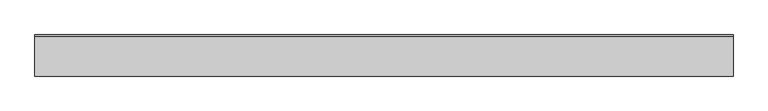
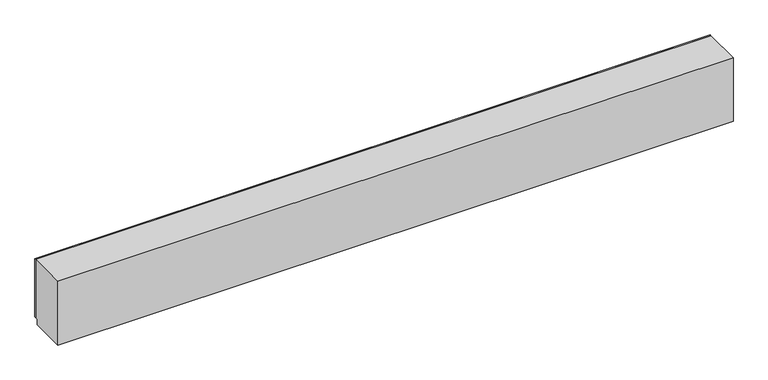
"""IFC4 building model written with IfcOpenShell, lengths in millimetres: furniture geometry, OD_CW_Base Cabinet : OD_CW_Base Cabinet."""

from ifc_helpers import new_model, si_unit, frame, origin, place, context, project, spatial, polyline, outline, extrude, source, transform, mapped, element, save


def furniture_ba198ac1(model_context):
    return source(origin(), model_context, "Body", "SweptSolid", [
        extrude(outline(polyline([(18.7377049, 82.55), (18.7377049, 107.95), (12195.519328, 107.95), (12195.519328, 82.55), (18.7377049, 82.55)])), frame((0.0, 0.0, 101.6), z_axis=(0.0, 0.0, 1.0), x_axis=(1.0, 0.0, 0.0)), (0.0, 0.0, 1.0), 1112.7587451),
        extrude(outline(polyline([(82.55, 1214.3587451), (82.55, 101.6), (31.75, 101.6), (31.75, 0.0), (-609.6, 0.0), (-609.6, 1214.3587451), (82.55, 1214.3587451)])), frame((18.7377049, 0.0, 0.0), z_axis=(1.0, 0.0, 0.0), x_axis=(0.0, 1.0, 0.0)), (0.0, 0.0, 1.0), 12176.7816231),
    ])


if __name__ == "__main__":
    model = new_model("IFC4")
    model_context = context("Model", 3, world=origin())
    ifc_project = project(units=[si_unit("LENGTHUNIT", "METRE", prefix="MILLI")], contexts=[model_context])
    site = spatial("IfcSite", under=ifc_project)
    building = spatial("IfcBuilding", under=site)
    placement = place(None, origin())
    furniture_shape = furniture_ba198ac1(model_context)
    element("IfcFurniture", 1, ObjectType="OD_CW_Base Cabinet : OD_CW_Base Cabinet", at=placement, inside=building, context=model_context, shape_type="MappedRepresentation", body=[
        mapped(furniture_shape, transform((0.0, 0.0, 0.0), x_axis=(1.0, 0.0, 0.0), y_axis=(0.0, 1.0, 0.0), z_axis=(0.0, 0.0, 1.0))),
    ])
    save(model, "model.ifc")

# Revit data of these elements
# Type "OD_CW_Base Cabinet : OD_CW_Base Cabinet"
#   OD_CW_Width [instance default] = 2' - 10"
#   OD_CW_Length [instance default] = 8' - 0"
#   OD_CW_Height [instance default] = 2' - 3"
#   Depth = 2' - 0"
#   Height = 3' - 0"
#   Width = 4' - 0"
#   OD_CW_Material_Front Panel [instance default] = none
#   OD_CW_Material_Body [instance default] = none
# Element 1 (IfcFurniture, "OD_CW_Base Cabinet : OD_CW_Base Cabinet")
#   OD_CW_Width = 2' - 4 1/4"
#   OD_CW_Length = 39' - 11.40085"
#   OD_CW_Height = 3' - 11.8094"
#   OD_CW_Material_Front Panel = WOOD-OAKFIRE
#   OD_CW_Material_Body = WHITE MARBLE COUNTERTOP
#   Materials on its faces: "WHITE MARBLE COUNTERTOP", "WOOD-OAKFIRE"
# Materials
#   "WHITE MARBLE COUNTERTOP": class "Wood", colour RGB 243 244 240, transparency 0, Description = "Generic wood", Cost = 0
#   "WOOD-OAKFIRE": class "Wood", colour RGB 198 202 183, transparency 0, Description = "Generic wood", Cost = 0
